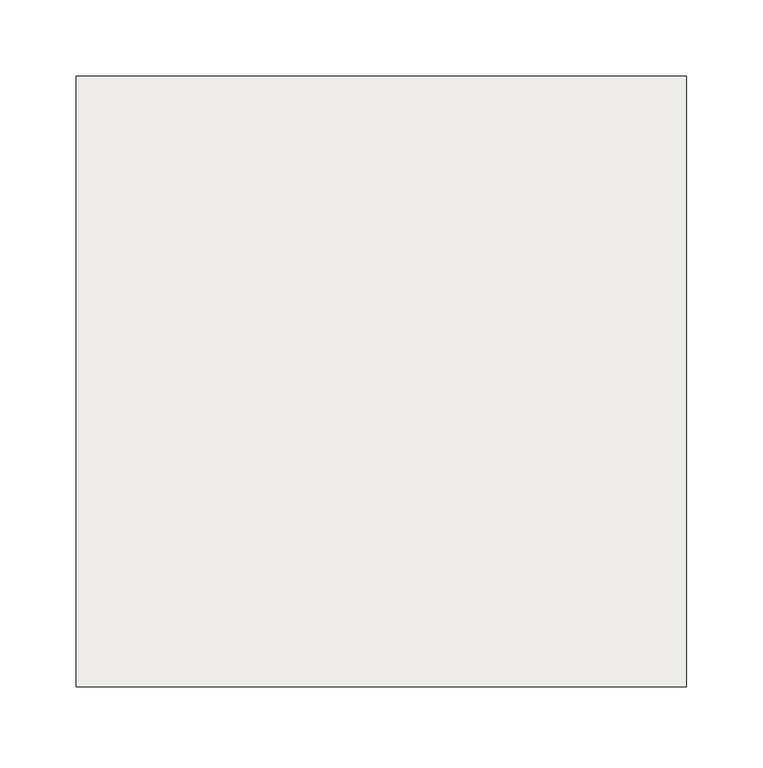
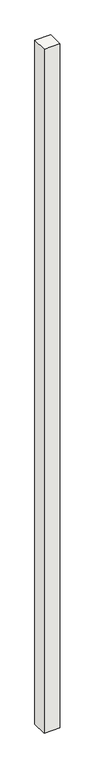
"""IFC4 building model written with IfcOpenShell, lengths in millimetres: slab geometry, NLRS_17_SFO_TLB_funderingspaal geheid beton prefab-AV-MMBPC_gen_rsf : heipaal beton prefab_gen__bxh 400x400."""

import ifcopenshell
import ifcopenshell.guid

model = None  # the IFC model being written
_history = None  # IfcOwnerHistory: only IFC2X3 demands one
_inside = {}  # id of a spatial element -> (the spatial element, [elements in it])
_under = {}  # id of a project, library or spatial element -> (it, [spatial elements below it])
_declared = {}  # id of a project -> (the project, [libraries it declares])
_typed = {}  # id of a type object -> (the type object, [elements of that type])
_made_of = {}  # id of a material, layer set ... -> (it, [elements and type objects made of it])


def new_model(schema):
    """Start an empty IFC model of exactly this schema.

    Asked for "IFC4X3", IfcOpenShell would pick the latest addendum, in which some entities
    have other attributes; the version numbers below select the first issue.
    IFC2X3 requires an IfcOwnerHistory on every rooted entity: one is made here for all.
    """
    global model, _history
    if schema == "IFC4X3":
        model = ifcopenshell.file(schema_version=(4, 3, 0, 0))
    else:
        model = ifcopenshell.file(schema=schema)
    _inside.clear()
    _under.clear()
    _declared.clear()
    _typed.clear()
    _made_of.clear()
    _history = None
    if model.schema == "IFC2X3":
        org = make("IfcOrganization", Name="unknown")
        user = make(
            "IfcPersonAndOrganization",
            ThePerson=make("IfcPerson", FamilyName="unknown"),
            TheOrganization=org,
        )
        app = make(
            "IfcApplication",
            ApplicationDeveloper=org,
            Version="unknown",
            ApplicationFullName="unknown",
            ApplicationIdentifier="unknown",
        )
        _history = make(
            "IfcOwnerHistory",
            OwningUser=user,
            OwningApplication=app,
            ChangeAction="ADDED",
            CreationDate=0,
        )
    return model


def make(cls, **values):
    """One entity of the class cls with the attributes given. An attribute that is None is left unset."""
    return model.create_entity(
        cls, **{name: value for name, value in values.items() if value is not None}
    )


def rooted(cls, **values):
    """An entity with a GlobalId (a new one), such as an element, a storey or a relation."""
    return make(cls, GlobalId=ifcopenshell.guid.new(), OwnerHistory=_history, **values)


def si_unit(unit_type, name, prefix=None):
    """IfcSIUnit, for example si_unit("LENGTHUNIT", "METRE", prefix="MILLI")."""
    return make("IfcSIUnit", UnitType=unit_type, Prefix=prefix, Name=name)


def assignment(units):
    """IfcUnitAssignment: the units of a project."""
    return None if units is None else make("IfcUnitAssignment", Units=units)


def point(xyz):
    """IfcCartesianPoint."""
    return None if xyz is None else make("IfcCartesianPoint", Coordinates=xyz)


def direction(xyz):
    """IfcDirection."""
    return None if xyz is None else make("IfcDirection", DirectionRatios=xyz)


def frame(location, z_axis=None, x_axis=None):
    """IfcAxis2Placement3D, a coordinate frame: its origin and axes. An axis left out is left unset."""
    return make(
        "IfcAxis2Placement3D",
        Location=point(location),
        Axis=direction(z_axis),
        RefDirection=direction(x_axis),
    )


def origin():
    """The frame at (0, 0, 0) with its axes left unset."""
    return frame((0.0, 0.0, 0.0))


def place(relative_to, where):
    """IfcLocalPlacement: puts the frame where relative to a parent placement (None: the world)."""
    return make(
        "IfcLocalPlacement", PlacementRelTo=relative_to, RelativePlacement=where
    )


def context(
    kind, dimensions, precision=None, world=None, true_north=None, identifier=None
):
    """IfcGeometricRepresentationContext, for example the 3D "Model" context."""
    return make(
        "IfcGeometricRepresentationContext",
        ContextIdentifier=identifier,
        ContextType=kind,
        CoordinateSpaceDimension=dimensions,
        Precision=precision,
        WorldCoordinateSystem=world,
        TrueNorth=true_north,
    )


def project(units=None, contexts=None):
    """IfcProject with its units and contexts."""
    return rooted(
        "IfcProject",
        Name="project",
        RepresentationContexts=contexts,
        UnitsInContext=assignment(units),
    )


def spatial(cls, under=None, at=None, **own):
    """A site, building, storey or space (cls), placed at a placement, below another one or the project."""
    s = rooted(cls, ObjectPlacement=at, **own)
    if under is not None:
        _under.setdefault(under.id(), (under, []))[1].append(s)
    return s


def polyline(points):
    """IfcPolyline through the points."""
    return make("IfcPolyline", Points=[point(p) for p in points])


def outline(outer, holes=None, kind="AREA"):
    """IfcArbitraryClosedProfileDef: a profile drawn as a closed curve; with holes, ...WithVoids."""
    if holes is None:
        return make("IfcArbitraryClosedProfileDef", ProfileType=kind, OuterCurve=outer)
    return make(
        "IfcArbitraryProfileDefWithVoids",
        ProfileType=kind,
        OuterCurve=outer,
        InnerCurves=holes,
    )


def extrude(swept, where, along, depth):
    """IfcExtrudedAreaSolid: the profile swept, set in the frame where, extruded along a direction by depth."""
    return make(
        "IfcExtrudedAreaSolid",
        SweptArea=swept,
        Position=where,
        ExtrudedDirection=direction(along),
        Depth=depth,
    )


def shape(context_of_items, identifier, shape_type, items):
    """IfcShapeRepresentation: the items that make up one representation, for example the "Body"."""
    return make(
        "IfcShapeRepresentation",
        ContextOfItems=context_of_items,
        RepresentationIdentifier=identifier,
        RepresentationType=shape_type,
        Items=items,
    )


def source(mapping_origin, context_of_items, identifier, shape_type, items):
    """IfcRepresentationMap: a shape defined once, which mapped items show again and again."""
    return make(
        "IfcRepresentationMap",
        MappingOrigin=mapping_origin,
        MappedRepresentation=shape(context_of_items, identifier, shape_type, items),
    )


def transform(
    local_origin,
    x_axis=None,
    y_axis=None,
    z_axis=None,
    scale=None,
    scale2=None,
    scale3=None,
    uniform=True,
):
    """IfcCartesianTransformationOperator3D, or its non-uniform kind. x_axis, y_axis, z_axis: its Axis1, 2, 3."""
    if uniform:
        return make(
            "IfcCartesianTransformationOperator3D",
            Axis1=direction(x_axis),
            Axis2=direction(y_axis),
            LocalOrigin=point(local_origin),
            Scale=scale,
            Axis3=direction(z_axis),
        )
    return make(
        "IfcCartesianTransformationOperator3DnonUniform",
        Axis1=direction(x_axis),
        Axis2=direction(y_axis),
        LocalOrigin=point(local_origin),
        Scale=scale,
        Axis3=direction(z_axis),
        Scale2=scale2,
        Scale3=scale3,
    )


def mapped(mapping_source, mapping_target):
    """IfcMappedItem: shows the shape of a source again, moved by a transform."""
    return make(
        "IfcMappedItem", MappingSource=mapping_source, MappingTarget=mapping_target
    )


def made_of(thing, what):
    """Note that an element or type object is made of a material, layer set ...; save() writes the relation."""
    if what is not None:
        _made_of.setdefault(what.id(), (what, []))[1].append(thing)
    return thing


def element(
    cls,
    number,
    at=None,
    inside=None,
    cuts=None,
    type_object=None,
    material=None,
    context=None,
    identifier="Body",
    shape_type=None,
    held_by="IfcProductDefinitionShape",
    body=None,
    shapes=None,
    **own,
):
    """One element of the class cls, such as IfcWall. Its Tag is "e" and its number.

    at: its placement. inside: the storey or other place that contains it. cuts: it is an
    opening in that element (IfcRelVoidsElement). A single representation is given by context,
    identifier, shape_type and body (its items); several are given by shapes. held_by: the class
    of the entity that holds the representations. save() writes the other relations.
    """
    e = rooted(cls, Tag="e%d" % number, ObjectPlacement=at, **own)
    if body is not None:
        shapes = [shape(context, identifier, shape_type, body)]
    if shapes is not None:
        e.Representation = make(held_by, Representations=shapes)
    if inside is not None:
        _inside.setdefault(inside.id(), (inside, []))[1].append(e)
    if cuts is not None:
        rooted(
            "IfcRelVoidsElement", RelatingBuildingElement=cuts, RelatedOpeningElement=e
        )
    if type_object is not None:
        _typed.setdefault(type_object.id(), (type_object, []))[1].append(e)
    return made_of(e, material)


def aggregate(whole, parts):
    """IfcRelAggregates: a whole, such as a stair, and the parts it consists of."""
    return rooted("IfcRelAggregates", RelatingObject=whole, RelatedObjects=parts)


def save(model, path):
    """Write the relations noted so far, then the file.

    IfcRelAggregates (storeys below a building ...), IfcRelContainedInSpatialStructure (elements
    in a storey), IfcRelDefinesByType, IfcRelAssociatesMaterial and IfcRelDeclares: one each for
    every whole, place, type object, material and project.
    """
    for whole, parts in _under.values():
        aggregate(whole, parts)
    for where, things in _inside.values():
        rooted(
            "IfcRelContainedInSpatialStructure",
            RelatedElements=things,
            RelatingStructure=where,
        )
    for kind, things in _typed.values():
        rooted("IfcRelDefinesByType", RelatedObjects=things, RelatingType=kind)
    for what, things in _made_of.values():
        rooted("IfcRelAssociatesMaterial", RelatedObjects=things, RelatingMaterial=what)
    for by, libraries in _declared.values():
        rooted("IfcRelDeclares", RelatingContext=by, RelatedDefinitions=libraries)
    model.write(path)


def slab_c32f4c5b(model_context):
    return source(origin(), model_context, "Body", "SweptSolid", [
        extrude(outline(polyline([(200.0, -200.0), (-200.0, -200.0), (-200.0, 200.0), (200.0, 200.0), (200.0, -200.0)])), frame((0.0, 0.0, -20000.0), z_axis=(0.0, 0.0, 1.0), x_axis=(1.0, 0.0, 0.0)), (0.0, 0.0, 1.0), 18290.0),
    ])


if __name__ == "__main__":
    model = new_model("IFC4")
    model_context = context("Model", 3, world=origin())
    ifc_project = project(units=[si_unit("LENGTHUNIT", "METRE", prefix="MILLI")], contexts=[model_context])
    site = spatial("IfcSite", under=ifc_project)
    building = spatial("IfcBuilding", under=site)
    placement = place(None, origin())
    slab_shape = slab_c32f4c5b(model_context)
    element("IfcSlab", 1, ObjectType="NLRS_17_SFO_TLB_funderingspaal geheid beton prefab-AV-MMBPC_gen_rsf : heipaal beton prefab_gen__bxh 400x400", at=placement, inside=building, context=model_context, shape_type="MappedRepresentation", body=[
        mapped(slab_shape, transform((0.0, 0.0, 0.0), x_axis=(1.0, 0.0, 0.0), y_axis=(0.0, 1.0, 0.0), z_axis=(0.0, 0.0, 1.0))),
    ])
    save(model, "model.ifc")

# Revit data of these elements
# Type "NLRS_17_SFO_TLB_funderingspaal geheid beton prefab-AV-MMBPC_gen_rsf : heipaal beton prefab_gen__bxh 400x400"
#   Export Type to IFC As = "IfcPile"
#   Type IfcGUID = "10$Kfo5uPCAOPJEOo5LE_W"
#   Type Comments = "prefab heipaal 400x400"
#   Model = " "
#   Manufacturer = " "
#   Description = "prefab heipaal 400x400"
#   Assembly Code = "17.21"
#   Width = 400 mm
#   Slanted Angle [instance default] = 0.00°
#   NLRS_S_draagvermogen_trek [instance default] = 0.00 kN
#   NLRS_S_draagvermogen_druk [instance default] = 0.00 kN
#   NLRS_C_lengte [instance default] = 1660 mm
#   NLRS_C_hoogte = 400 mm
#   NLRS_C_breedte = 400 mm
#   Height [instance default] = 1660 mm
#   Length [instance default] = 1660 mm
#   Angle [instance default] = 0.00°
#   Slanted [instance default] = 0
#   Structural Material = NLRS_f2_beton prefab_gen_rsf
#   Keynote = ""
# Element 1 (IfcSlab, "NLRS_17_SFO_TLB_funderingspaal geheid beton prefab-AV-MMBPC_gen_rsf : heipaal beton prefab_gen__bxh 400x400")
#   NLRS_C_lengte = 18290 mm
#   Height = 18290 mm
#   Length = 18290 mm
#   Materials on its faces: "NLRS_f2_beton prefab_gen_rsf"
# Materials
#   "NLRS_f2_beton prefab_gen_rsf": class "F - Niet gebakken kunststeen", colour RGB 129 133 118, transparency 0, Keynote = "f2", Manufacturer = "Revit Standards Foundation", URL = "www.revitstandards.org", Description = "beton prefab", Cost = 0
